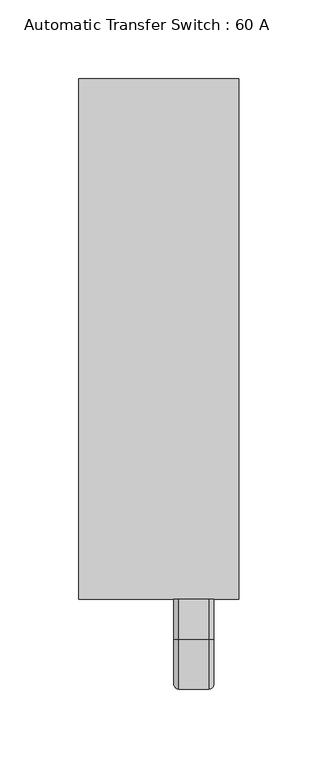
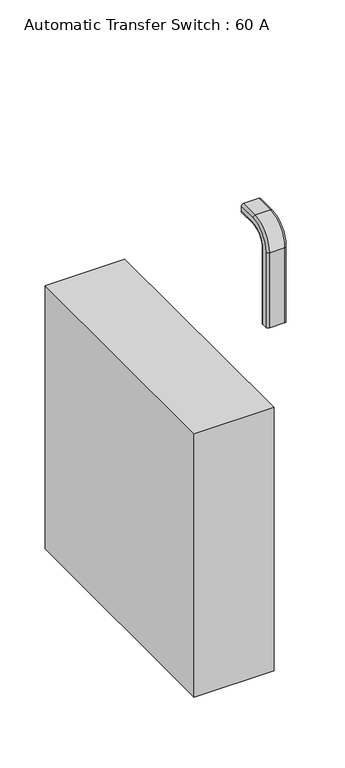
"""IFC4 building model written with IfcOpenShell, lengths in millimetres: proxy geometry, Automatic Transfer Switch : 60 A."""

from ifc_helpers import new_model, si_unit, point, frame, origin, origin_with_axes, place, context, project, spatial, polyline, circle_curve, ellipse_curve, trimmed, outline, extrude, source, transform, mapped, element, save
from ifc_brep_helpers import plane_surface, cylinder_surface, revolved_surface, advanced_brep


def automatic_transfer_switch_60_a_503ee7c5(model_context):
    return source(origin(), model_context, "Body", "SolidModel", [
        extrude(outline(polyline([(50.8, 0.0), (50.8, -330.2), (-50.8, -330.2), (-50.8, 0.0), (50.8, 0.0)])), origin_with_axes(), (0.0, 0.0, 1.0), 355.6),
        advanced_brep(
        [(12.7, -330.2, 644.525), (31.7743566, -330.2, 644.525), (34.9493566, -330.2, 641.35), (34.9493566, -330.2, 635.2833203), (31.7743566, -330.2, 631.825), (12.7, -330.2, 631.825), (9.525, -330.2, 635.0), (9.525, -330.2, 641.35), (12.7, -355.6, 644.525), (31.7743566, -355.6, 644.525), (34.9493566, -355.6, 641.35), (34.9493566, -384.175, 612.775), (34.9493566, -384.175, 511.175), (34.9493566, -378.1083203, 511.175), (34.9493566, -378.1083203, 612.775), (34.9493566, -355.6, 635.2833203), (31.7743566, -355.6, 631.825), (12.7, -355.6, 631.825), (9.525, -355.6, 635.0), (9.525, -377.825, 612.775), (9.525, -377.825, 511.175), (9.525, -384.175, 511.175), (9.525, -384.175, 612.775), (9.525, -355.6, 641.35), (31.7743566, -387.35, 612.775), (12.7, -387.35, 612.775), (31.7743566, -374.65, 612.775), (12.7, -374.65, 612.775), (12.7, -387.35, 511.175), (12.7, -374.65, 511.175), (31.7743566, -374.65, 511.175), (31.7743566, -387.35, 511.175)],
        [
            (0, 1),
            (1, 2, circle_curve(frame((31.7743566, -330.2, 641.35), z_axis=(0.0, 1.0, 0.0), x_axis=(0.0, 0.0, -1.0)), 3.175)),
            (2, 3),
            (3, 4, circle_curve(frame((31.7743566, -330.2, 635.0116054), z_axis=(0.0, 1.0, 0.0), x_axis=(0.0, 0.0, -1.0)), 3.1866054)),
            (4, 5),
            (5, 6, circle_curve(frame((12.7, -330.2, 635.0), z_axis=(0.0, 1.0, 0.0), x_axis=(0.0, 0.0, -1.0)), 3.175)),
            (6, 7),
            (7, 0, circle_curve(frame((12.7, -330.2, 641.35), z_axis=(0.0, 1.0, 0.0), x_axis=(0.0, 0.0, -1.0)), 3.175)),
            (0, 8),
            (8, 9),
            (9, 1),
            (9, 10, circle_curve(frame((31.7743566, -355.6, 641.35), z_axis=(0.0, 1.0, 0.0), x_axis=(0.0, 0.0, -1.0)), 3.175)),
            (10, 2),
            (10, 11, circle_curve(frame((34.9493566, -355.6, 612.775), z_axis=(1.0, 0.0, 0.0), x_axis=(0.0, 0.0, 1.0)), 28.575)),
            (11, 12),
            (12, 13),
            (13, 14),
            (14, 15, circle_curve(frame((34.9493566, -355.6, 612.775), z_axis=(-1.0, 0.0, 0.0), x_axis=(0.0, 0.0, 1.0)), 22.5083203)),
            (15, 3),
            (15, 16, circle_curve(frame((31.7743566, -355.6, 635.0116054), z_axis=(0.0, 1.0, 0.0), x_axis=(0.0, 0.0, -1.0)), 3.1866054)),
            (16, 4),
            (16, 17),
            (17, 5),
            (17, 18, circle_curve(frame((12.7, -355.6, 635.0), z_axis=(0.0, 1.0, 0.0), x_axis=(0.0, 0.0, -1.0)), 3.175)),
            (18, 6),
            (18, 19, circle_curve(frame((9.525, -355.6, 612.775), z_axis=(1.0, 0.0, 0.0), x_axis=(0.0, 0.0, 1.0)), 22.225)),
            (19, 20),
            (20, 21),
            (21, 22),
            (22, 23, circle_curve(frame((9.525, -355.6, 612.775), z_axis=(-1.0, 0.0, 0.0), x_axis=(0.0, 0.0, 1.0)), 28.575)),
            (23, 7),
            (23, 8, circle_curve(frame((12.7, -355.6, 641.35), z_axis=(0.0, 1.0, 0.0), x_axis=(0.0, 0.0, -1.0)), 3.175)),
            (24, 9, circle_curve(frame((31.7743566, -355.6, 612.775), z_axis=(-1.0, 0.0, 0.0), x_axis=(0.0, 0.0, 1.0)), 31.75)),
            (8, 25, circle_curve(frame((12.7, -355.6, 612.775), z_axis=(1.0, 0.0, 0.0), x_axis=(0.0, 0.0, 1.0)), 31.75)),
            (25, 24),
            (24, 11, circle_curve(frame((31.7743566, -384.175, 612.775), z_axis=(0.0, 0.0, 1.0), x_axis=(0.0, 1.0, 0.0)), 3.175)),
            (26, 16, circle_curve(frame((31.7743566, -355.6, 612.775), z_axis=(-1.0, 0.0, 0.0), x_axis=(0.0, 0.0, 1.0)), 19.05)),
            (14, 26, circle_curve(frame((31.7743566, -377.8366054, 612.775), z_axis=(0.0, 0.0, 1.0), x_axis=(0.0, 1.0, 0.0)), 3.1866054)),
            (27, 17, circle_curve(frame((12.7, -355.6, 612.775), z_axis=(-1.0, 0.0, 0.0), x_axis=(0.0, 0.0, 1.0)), 19.05)),
            (26, 27),
            (27, 19, circle_curve(frame((12.7, -377.825, 612.775), z_axis=(0.0, 0.0, 1.0), x_axis=(0.0, 1.0, 0.0)), 3.175)),
            (22, 25, circle_curve(frame((12.7, -384.175, 612.775), z_axis=(0.0, 0.0, 1.0), x_axis=(0.0, 1.0, 0.0)), 3.175)),
            (28, 21, circle_curve(frame((12.7, -384.175, 511.175), z_axis=(0.0, 0.0, -1.0), x_axis=(0.0, 1.0, 0.0)), 3.175)),
            (20, 29, circle_curve(frame((12.7, -377.825, 511.175), z_axis=(0.0, 0.0, -1.0), x_axis=(0.0, 1.0, 0.0)), 3.175)),
            (29, 30),
            (30, 13, circle_curve(frame((31.7743566, -377.8366054, 511.175), z_axis=(0.0, 0.0, -1.0), x_axis=(0.0, 1.0, 0.0)), 3.1866054)),
            (12, 31, circle_curve(frame((31.7743566, -384.175, 511.175), z_axis=(0.0, 0.0, -1.0), x_axis=(0.0, 1.0, 0.0)), 3.175)),
            (31, 28),
            (25, 28),
            (31, 24),
            (30, 26),
            (29, 27),
        ],
        [
            plane_surface(frame((22.225, -330.2, 638.175), z_axis=(0.0, 1.0, 0.0), x_axis=(1.0, 0.0, 0.0))),
            plane_surface(frame((12.7, -330.2, 644.525), z_axis=(0.0, 0.0, 1.0), x_axis=(0.0, -1.0, 0.0))),
            cylinder_surface(frame((31.7743566, -330.2, 641.35), z_axis=(0.0, 1.0, 0.0), x_axis=(0.0, 0.0, -1.0)), 3.175),
            plane_surface(frame((34.9493566, -330.2, 641.35), z_axis=(1.0, 0.0, 0.0), x_axis=(0.0, -1.0, 0.0))),
            cylinder_surface(frame((31.7743566, -330.2, 635.0116054), z_axis=(0.0, 1.0, 0.0), x_axis=(0.0, 0.0, -1.0)), 3.1866054),
            plane_surface(frame((31.7743566, -330.2, 631.825), z_axis=(0.0, 0.0, -1.0), x_axis=(0.0, -1.0, 0.0))),
            cylinder_surface(frame((12.7, -330.2, 635.0), z_axis=(0.0, 1.0, 0.0), x_axis=(0.0, 0.0, -1.0)), 3.175),
            plane_surface(frame((9.525, -330.2, 635.0), z_axis=(-1.0, 0.0, 0.0), x_axis=(0.0, -1.0, 0.0))),
            cylinder_surface(frame((12.7, -330.2, 641.35), z_axis=(0.0, 1.0, 0.0), x_axis=(0.0, 0.0, -1.0)), 3.175),
            cylinder_surface(frame((22.225, -355.6, 612.775), z_axis=(1.0, 0.0, 0.0), x_axis=(0.0, 0.0, 1.0)), 31.75),
            revolved_surface(trimmed(ellipse_curve(frame((31.7743566, -355.6, 641.35), z_axis=(0.0, 1.0, 0.0), x_axis=(0.0, 0.0, -1.0)), 3.175, 3.175), [point((31.7743566, -355.6, 644.525))], [point((34.9493566, -355.6, 641.35))], True, "CARTESIAN"), (22.225, -355.6, 612.775), (1.0, 0.0, 0.0)),
            revolved_surface(trimmed(ellipse_curve(frame((31.7743566, -355.6, 635.0116054), z_axis=(0.0, 1.0, 0.0), x_axis=(0.0, 0.0, -1.0)), 3.1866054, 3.1866054), [point((34.9493566, -355.6, 635.2833203))], [point((31.7743566, -355.6, 631.825))], True, "CARTESIAN"), (22.225, -355.6, 612.775), (1.0, 0.0, 0.0)),
            revolved_surface(polyline([(31.7743566, -355.6, 631.8249999999999), (12.7, -355.6, 631.8249999999999)]), (22.225, -355.6, 612.775), (1.0, 0.0, 0.0)),
            revolved_surface(trimmed(ellipse_curve(frame((12.7, -355.6, 635.0), z_axis=(0.0, 1.0, 0.0), x_axis=(0.0, 0.0, -1.0)), 3.175, 3.175), [point((12.7, -355.6, 631.825))], [point((9.525, -355.6, 635.0))], True, "CARTESIAN"), (22.225, -355.6, 612.775), (1.0, 0.0, 0.0)),
            revolved_surface(trimmed(ellipse_curve(frame((12.7, -355.6, 641.35), z_axis=(0.0, 1.0, 0.0), x_axis=(0.0, 0.0, -1.0)), 3.175, 3.175), [point((9.525, -355.6, 641.35))], [point((12.7, -355.6, 644.525))], True, "CARTESIAN"), (22.225, -355.6, 612.775), (1.0, 0.0, 0.0)),
            plane_surface(frame((22.225, -381.0, 511.175), z_axis=(0.0, 0.0, -1.0), x_axis=(1.0, 0.0, 0.0))),
            plane_surface(frame((12.7, -387.35, 612.775), z_axis=(0.0, -1.0, 0.0), x_axis=(0.0, 0.0, -1.0))),
            cylinder_surface(frame((31.7743566, -384.175, 612.775), z_axis=(0.0, 0.0, 1.0), x_axis=(0.0, 1.0, 0.0)), 3.175),
            cylinder_surface(frame((31.7743566, -377.8366054, 612.775), z_axis=(0.0, 0.0, 1.0), x_axis=(0.0, 1.0, 0.0)), 3.1866054),
            plane_surface(frame((31.7743566, -374.65, 612.775), z_axis=(0.0, 1.0, 0.0), x_axis=(0.0, 0.0, -1.0))),
            cylinder_surface(frame((12.7, -377.825, 612.775), z_axis=(0.0, 0.0, 1.0), x_axis=(0.0, 1.0, 0.0)), 3.175),
            cylinder_surface(frame((12.7, -384.175, 612.775), z_axis=(0.0, 0.0, 1.0), x_axis=(0.0, 1.0, 0.0)), 3.175),
        ],
        [
            (0, [[1, 2, 3, 4, 5, 6, 7, 8]]),
            (1, [[-1, 9, 10, 11]]),
            (2, [[-2, -11, 12, 13]]),
            (3, [[-3, -13, 14, 15, 16, 17, 18, 19]]),
            (4, [[-4, -19, 20, 21]]),
            (5, [[-5, -21, 22, 23]]),
            (6, [[-6, -23, 24, 25]]),
            (7, [[-7, -25, 26, 27, 28, 29, 30, 31]]),
            (8, [[-8, -31, 32, -9]]),
            (9, [[33, -10, 34, 35]]),
            (10, [[-14, -12, -33, 36]]),
            (11, [[37, -20, -18, 38]]),
            (12, [[39, -22, -37, 40]]),
            (13, [[-26, -24, -39, 41]]),
            (14, [[-34, -32, -30, 42]]),
            (15, [[43, -28, 44, 45, 46, -16, 47, 48]]),
            (16, [[-35, 49, -48, 50]]),
            (17, [[-36, -50, -47, -15]]),
            (18, [[-38, -17, -46, 51]]),
            (19, [[-40, -51, -45, 52]]),
            (20, [[-41, -52, -44, -27]]),
            (21, [[-42, -29, -43, -49]]),
        ],
    ),
    ])


if __name__ == "__main__":
    model = new_model("IFC4")
    model_context = context("Model", 3, world=origin())
    ifc_project = project(units=[si_unit("LENGTHUNIT", "METRE", prefix="MILLI")], contexts=[model_context])
    site = spatial("IfcSite", under=ifc_project)
    building = spatial("IfcBuilding", under=site)
    placement = place(None, origin())
    automatic_transfer_switch_60_a_shape = automatic_transfer_switch_60_a_503ee7c5(model_context)
    element("IfcBuildingElementProxy", 1, Name="Automatic Transfer Switch : 60 A", ObjectType="Automatic Transfer Switch : 60 A", at=placement, inside=building, context=model_context, shape_type="MappedRepresentation", body=[
        mapped(automatic_transfer_switch_60_a_shape, transform((0.0, 0.0, 0.0), x_axis=(1.0, 0.0, 0.0), y_axis=(0.0, 1.0, 0.0), z_axis=(0.0, 0.0, 1.0))),
    ])
    save(model, "model.ifc")

# Revit data of these elements
# Type "Automatic Transfer Switch : 60 A"
#   COBie.Type.CreatedBy = "design@eagle.com"
#   COBie.Type.CreatedOn = "2016-10-27T05:31:12"
#   COBie.Type.Name = "Automatic Transfer Switch_60 A"
#   COBie.Type.Category = "23-80 30 11 17 : Distribution Boards and Control Panels"
#   COBie.Type.Description = "Automatic Transfer Switch_60 A"
#   COBie.Type.Manufacturer = ""
#   COBie.Type.ModelNumber = ""
#   COBie.Type.ReplacementCost = 0
#   Width 2 = 0' - 7 5/8"
#   Width 1 = 0' - 2 7/8"
#   Switch Width = 1' - 3 1/4"
#   Switch Voltage = 240 V
#   Switch Length = 0' - 4"
#   Switch Height = 1' - 2"
#   Length 1 = 0' - 2"
#   Height 1 = 1' - 10 3/4"
#   COBie.Type = yes
#   Number of Poles = 2
#   Switch Material = none
#   Load Classification = Other
